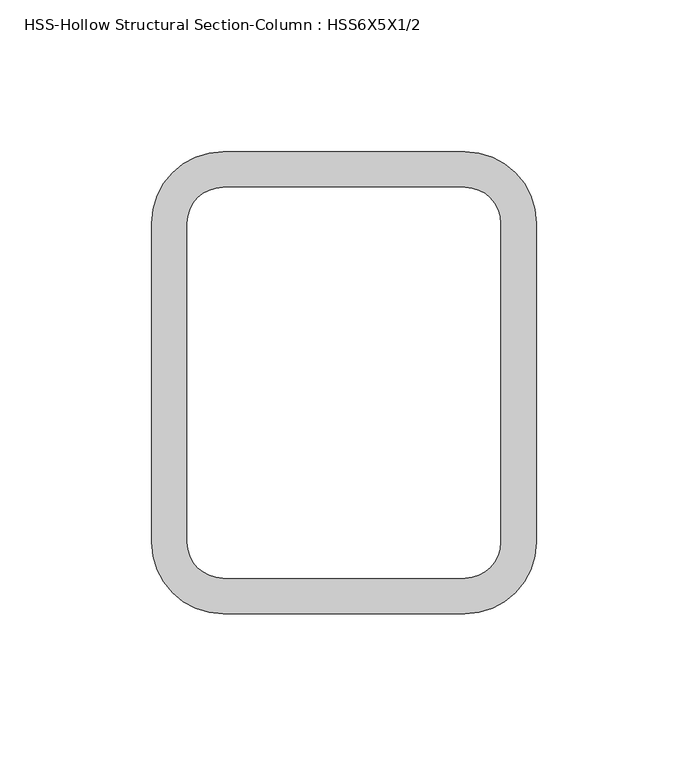
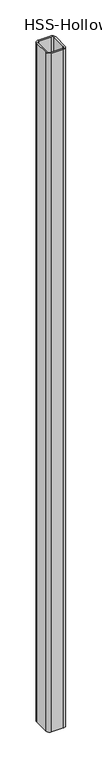
"""IFC4 building model written with IfcOpenShell, lengths in millimetres: column geometry, HSS-Hollow Structural Section-Column : HSS6X5X1/2."""

import ifcopenshell
import ifcopenshell.guid

model = None  # the IFC model being written
_history = None  # IfcOwnerHistory: only IFC2X3 demands one
_inside = {}  # id of a spatial element -> (the spatial element, [elements in it])
_under = {}  # id of a project, library or spatial element -> (it, [spatial elements below it])
_declared = {}  # id of a project -> (the project, [libraries it declares])
_typed = {}  # id of a type object -> (the type object, [elements of that type])
_made_of = {}  # id of a material, layer set ... -> (it, [elements and type objects made of it])


def new_model(schema):
    """Start an empty IFC model of exactly this schema.

    Asked for "IFC4X3", IfcOpenShell would pick the latest addendum, in which some entities
    have other attributes; the version numbers below select the first issue.
    IFC2X3 requires an IfcOwnerHistory on every rooted entity: one is made here for all.
    """
    global model, _history
    if schema == "IFC4X3":
        model = ifcopenshell.file(schema_version=(4, 3, 0, 0))
    else:
        model = ifcopenshell.file(schema=schema)
    _inside.clear()
    _under.clear()
    _declared.clear()
    _typed.clear()
    _made_of.clear()
    _history = None
    if model.schema == "IFC2X3":
        org = make("IfcOrganization", Name="unknown")
        user = make(
            "IfcPersonAndOrganization",
            ThePerson=make("IfcPerson", FamilyName="unknown"),
            TheOrganization=org,
        )
        app = make(
            "IfcApplication",
            ApplicationDeveloper=org,
            Version="unknown",
            ApplicationFullName="unknown",
            ApplicationIdentifier="unknown",
        )
        _history = make(
            "IfcOwnerHistory",
            OwningUser=user,
            OwningApplication=app,
            ChangeAction="ADDED",
            CreationDate=0,
        )
    return model


def make(cls, **values):
    """One entity of the class cls with the attributes given. An attribute that is None is left unset."""
    return model.create_entity(
        cls, **{name: value for name, value in values.items() if value is not None}
    )


def rooted(cls, **values):
    """An entity with a GlobalId (a new one), such as an element, a storey or a relation."""
    return make(cls, GlobalId=ifcopenshell.guid.new(), OwnerHistory=_history, **values)


def si_unit(unit_type, name, prefix=None):
    """IfcSIUnit, for example si_unit("LENGTHUNIT", "METRE", prefix="MILLI")."""
    return make("IfcSIUnit", UnitType=unit_type, Prefix=prefix, Name=name)


def assignment(units):
    """IfcUnitAssignment: the units of a project."""
    return None if units is None else make("IfcUnitAssignment", Units=units)


def point(xyz):
    """IfcCartesianPoint."""
    return None if xyz is None else make("IfcCartesianPoint", Coordinates=xyz)


def direction(xyz):
    """IfcDirection."""
    return None if xyz is None else make("IfcDirection", DirectionRatios=xyz)


def frame(location, z_axis=None, x_axis=None):
    """IfcAxis2Placement3D, a coordinate frame: its origin and axes. An axis left out is left unset."""
    return make(
        "IfcAxis2Placement3D",
        Location=point(location),
        Axis=direction(z_axis),
        RefDirection=direction(x_axis),
    )


def frame_2d(location, x_axis=None):
    """IfcAxis2Placement2D, a coordinate frame in the plane: its origin and x axis."""
    return make(
        "IfcAxis2Placement2D", Location=point(location), RefDirection=direction(x_axis)
    )


def origin():
    """The frame at (0, 0, 0) with its axes left unset."""
    return frame((0.0, 0.0, 0.0))


def place(relative_to, where):
    """IfcLocalPlacement: puts the frame where relative to a parent placement (None: the world)."""
    return make(
        "IfcLocalPlacement", PlacementRelTo=relative_to, RelativePlacement=where
    )


def context(
    kind, dimensions, precision=None, world=None, true_north=None, identifier=None
):
    """IfcGeometricRepresentationContext, for example the 3D "Model" context."""
    return make(
        "IfcGeometricRepresentationContext",
        ContextIdentifier=identifier,
        ContextType=kind,
        CoordinateSpaceDimension=dimensions,
        Precision=precision,
        WorldCoordinateSystem=world,
        TrueNorth=true_north,
    )


def project(units=None, contexts=None):
    """IfcProject with its units and contexts."""
    return rooted(
        "IfcProject",
        Name="project",
        RepresentationContexts=contexts,
        UnitsInContext=assignment(units),
    )


def spatial(cls, under=None, at=None, **own):
    """A site, building, storey or space (cls), placed at a placement, below another one or the project."""
    s = rooted(cls, ObjectPlacement=at, **own)
    if under is not None:
        _under.setdefault(under.id(), (under, []))[1].append(s)
    return s


def polyline(points):
    """IfcPolyline through the points."""
    return make("IfcPolyline", Points=[point(p) for p in points])


def circle_curve(where, radius):
    """IfcCircle in the frame where."""
    return make("IfcCircle", Position=where, Radius=radius)


def trimmed(basis, trim1, trim2, sense, master):
    """IfcTrimmedCurve: the piece of a basis curve between two trims."""
    return make(
        "IfcTrimmedCurve",
        BasisCurve=basis,
        Trim1=trim1,
        Trim2=trim2,
        SenseAgreement=sense,
        MasterRepresentation=master,
    )


def segment(curve, same_sense, transition):
    """IfcCompositeCurveSegment."""
    return make(
        "IfcCompositeCurveSegment",
        Transition=transition,
        SameSense=same_sense,
        ParentCurve=curve,
    )


def composite_curve(segments, self_intersect=None):
    """IfcCompositeCurve: segments joined end to end."""
    return make("IfcCompositeCurve", Segments=segments, SelfIntersect=self_intersect)


def outline(outer, holes=None, kind="AREA"):
    """IfcArbitraryClosedProfileDef: a profile drawn as a closed curve; with holes, ...WithVoids."""
    if holes is None:
        return make("IfcArbitraryClosedProfileDef", ProfileType=kind, OuterCurve=outer)
    return make(
        "IfcArbitraryProfileDefWithVoids",
        ProfileType=kind,
        OuterCurve=outer,
        InnerCurves=holes,
    )


def extrude(swept, where, along, depth):
    """IfcExtrudedAreaSolid: the profile swept, set in the frame where, extruded along a direction by depth."""
    return make(
        "IfcExtrudedAreaSolid",
        SweptArea=swept,
        Position=where,
        ExtrudedDirection=direction(along),
        Depth=depth,
    )


def shape(context_of_items, identifier, shape_type, items):
    """IfcShapeRepresentation: the items that make up one representation, for example the "Body"."""
    return make(
        "IfcShapeRepresentation",
        ContextOfItems=context_of_items,
        RepresentationIdentifier=identifier,
        RepresentationType=shape_type,
        Items=items,
    )


def source(mapping_origin, context_of_items, identifier, shape_type, items):
    """IfcRepresentationMap: a shape defined once, which mapped items show again and again."""
    return make(
        "IfcRepresentationMap",
        MappingOrigin=mapping_origin,
        MappedRepresentation=shape(context_of_items, identifier, shape_type, items),
    )


def transform(
    local_origin,
    x_axis=None,
    y_axis=None,
    z_axis=None,
    scale=None,
    scale2=None,
    scale3=None,
    uniform=True,
):
    """IfcCartesianTransformationOperator3D, or its non-uniform kind. x_axis, y_axis, z_axis: its Axis1, 2, 3."""
    if uniform:
        return make(
            "IfcCartesianTransformationOperator3D",
            Axis1=direction(x_axis),
            Axis2=direction(y_axis),
            LocalOrigin=point(local_origin),
            Scale=scale,
            Axis3=direction(z_axis),
        )
    return make(
        "IfcCartesianTransformationOperator3DnonUniform",
        Axis1=direction(x_axis),
        Axis2=direction(y_axis),
        LocalOrigin=point(local_origin),
        Scale=scale,
        Axis3=direction(z_axis),
        Scale2=scale2,
        Scale3=scale3,
    )


def mapped(mapping_source, mapping_target):
    """IfcMappedItem: shows the shape of a source again, moved by a transform."""
    return make(
        "IfcMappedItem", MappingSource=mapping_source, MappingTarget=mapping_target
    )


def made_of(thing, what):
    """Note that an element or type object is made of a material, layer set ...; save() writes the relation."""
    if what is not None:
        _made_of.setdefault(what.id(), (what, []))[1].append(thing)
    return thing


def element(
    cls,
    number,
    at=None,
    inside=None,
    cuts=None,
    type_object=None,
    material=None,
    context=None,
    identifier="Body",
    shape_type=None,
    held_by="IfcProductDefinitionShape",
    body=None,
    shapes=None,
    **own,
):
    """One element of the class cls, such as IfcWall. Its Tag is "e" and its number.

    at: its placement. inside: the storey or other place that contains it. cuts: it is an
    opening in that element (IfcRelVoidsElement). A single representation is given by context,
    identifier, shape_type and body (its items); several are given by shapes. held_by: the class
    of the entity that holds the representations. save() writes the other relations.
    """
    e = rooted(cls, Tag="e%d" % number, ObjectPlacement=at, **own)
    if body is not None:
        shapes = [shape(context, identifier, shape_type, body)]
    if shapes is not None:
        e.Representation = make(held_by, Representations=shapes)
    if inside is not None:
        _inside.setdefault(inside.id(), (inside, []))[1].append(e)
    if cuts is not None:
        rooted(
            "IfcRelVoidsElement", RelatingBuildingElement=cuts, RelatedOpeningElement=e
        )
    if type_object is not None:
        _typed.setdefault(type_object.id(), (type_object, []))[1].append(e)
    return made_of(e, material)


def aggregate(whole, parts):
    """IfcRelAggregates: a whole, such as a stair, and the parts it consists of."""
    return rooted("IfcRelAggregates", RelatingObject=whole, RelatedObjects=parts)


def save(model, path):
    """Write the relations noted so far, then the file.

    IfcRelAggregates (storeys below a building ...), IfcRelContainedInSpatialStructure (elements
    in a storey), IfcRelDefinesByType, IfcRelAssociatesMaterial and IfcRelDeclares: one each for
    every whole, place, type object, material and project.
    """
    for whole, parts in _under.values():
        aggregate(whole, parts)
    for where, things in _inside.values():
        rooted(
            "IfcRelContainedInSpatialStructure",
            RelatedElements=things,
            RelatingStructure=where,
        )
    for kind, things in _typed.values():
        rooted("IfcRelDefinesByType", RelatedObjects=things, RelatingType=kind)
    for what, things in _made_of.values():
        rooted("IfcRelAssociatesMaterial", RelatedObjects=things, RelatingMaterial=what)
    for by, libraries in _declared.values():
        rooted("IfcRelDeclares", RelatingContext=by, RelatedDefinitions=libraries)
    model.write(path)


def hss_hollow_structural_section_column_hss6x5x1_2_1fd848d0(model_context):
    return source(origin(), model_context, "Body", "SweptSolid", [
        extrude(outline(composite_curve([segment(trimmed(circle_curve(frame_2d((39.878, 52.578)), 23.622), [point((39.878, 76.2))], [point((63.5, 52.578))], False, "CARTESIAN"), True, "CONTINUOUS"), segment(polyline([(63.5, 52.578), (63.5, -52.578)]), True, "CONTINUOUS"), segment(trimmed(circle_curve(frame_2d((39.878, -52.578)), 23.622), [point((63.5, -52.578))], [point((39.878, -76.2))], False, "CARTESIAN"), True, "CONTINUOUS"), segment(polyline([(39.878, -76.2), (-39.878, -76.2)]), True, "CONTINUOUS"), segment(trimmed(circle_curve(frame_2d((-39.878, -52.578)), 23.622), [point((-39.878, -76.2))], [point((-63.5, -52.578))], False, "CARTESIAN"), True, "CONTINUOUS"), segment(polyline([(-63.5, -52.578), (-63.5, 52.578)]), True, "CONTINUOUS"), segment(trimmed(circle_curve(frame_2d((-39.878, 52.578)), 23.622), [point((-63.5, 52.578))], [point((-39.878, 76.2))], False, "CARTESIAN"), True, "CONTINUOUS"), segment(polyline([(-39.878, 76.2), (39.878, 76.2)]), True, "CONTINUOUS")], self_intersect=False), holes=[composite_curve([segment(polyline([(39.878, 64.389), (-39.878, 64.389)]), True, "CONTINUOUS"), segment(trimmed(circle_curve(frame_2d((-39.878, 52.578)), 11.811), [point((-39.878, 64.389))], [point((-51.689, 52.578))], True, "CARTESIAN"), True, "CONTINUOUS"), segment(polyline([(-51.689, 52.578), (-51.689, -52.578)]), True, "CONTINUOUS"), segment(trimmed(circle_curve(frame_2d((-39.878, -52.578)), 11.811), [point((-51.689, -52.578))], [point((-39.878, -64.389))], True, "CARTESIAN"), True, "CONTINUOUS"), segment(polyline([(-39.878, -64.389), (39.878, -64.389)]), True, "CONTINUOUS"), segment(trimmed(circle_curve(frame_2d((39.878, -52.578)), 11.811), [point((39.878, -64.389))], [point((51.689, -52.578))], True, "CARTESIAN"), True, "CONTINUOUS"), segment(polyline([(51.689, -52.578), (51.689, 52.578)]), True, "CONTINUOUS"), segment(trimmed(circle_curve(frame_2d((39.878, 52.578)), 11.811), [point((51.689, 52.578))], [point((39.878, 64.389))], True, "CARTESIAN"), True, "CONTINUOUS")], self_intersect=False)]), frame((0.0, 0.0, -304.8), z_axis=(0.0, 0.0, 1.0), x_axis=(1.0, 0.0, 0.0)), (0.0, 0.0, 1.0), 4775.2),
    ])


if __name__ == "__main__":
    model = new_model("IFC4")
    model_context = context("Model", 3, world=origin())
    ifc_project = project(units=[si_unit("LENGTHUNIT", "METRE", prefix="MILLI")], contexts=[model_context])
    site = spatial("IfcSite", under=ifc_project)
    building = spatial("IfcBuilding", under=site)
    placement = place(None, origin())
    hss_hollow_structural_section_column_hss6x5x1_2_shape = hss_hollow_structural_section_column_hss6x5x1_2_1fd848d0(model_context)
    element("IfcColumn", 1, ObjectType="HSS-Hollow Structural Section-Column : HSS6X5X1/2", at=placement, inside=building, context=model_context, shape_type="MappedRepresentation", body=[
        mapped(hss_hollow_structural_section_column_hss6x5x1_2_shape, transform((0.0, 0.0, 0.0), x_axis=(1.0, 0.0, 0.0), y_axis=(0.0, 1.0, 0.0), z_axis=(0.0, 0.0, 1.0))),
    ])
    save(model, "model.ifc")

# Revit data of these elements
# Type "HSS-Hollow Structural Section-Column : HSS6X5X1/2"
#   Assembly Code = "B10"
#   Shape = "Rect."
#   W = 31.7
#   Ht = 0' - 6"
#   b = 0' - 5"
#   kr = 0' - 0.93"
#   t = 0' - 0.465"
#   A = 0.0611806 SF
#   Structural Material [instance default] = Steel ASTM A500, Grade B, Rectangular and Square
# Element 1 (IfcColumn, "HSS-Hollow Structural Section-Column : HSS6X5X1/2")
#   Structural Material = Metal - Steel - ASTM A992
#   Materials on its faces: "Metal - Steel - ASTM A992"
# Materials
#   "Steel ASTM A500, Grade B, Rectangular and Square": class "Metal", colour RGB 199 199 199, transparency 0, Description = "Carbon steel", Cost = 0
#   "Metal - Steel - ASTM A992": class "Metal", colour RGB 255 128 0, transparency 0
